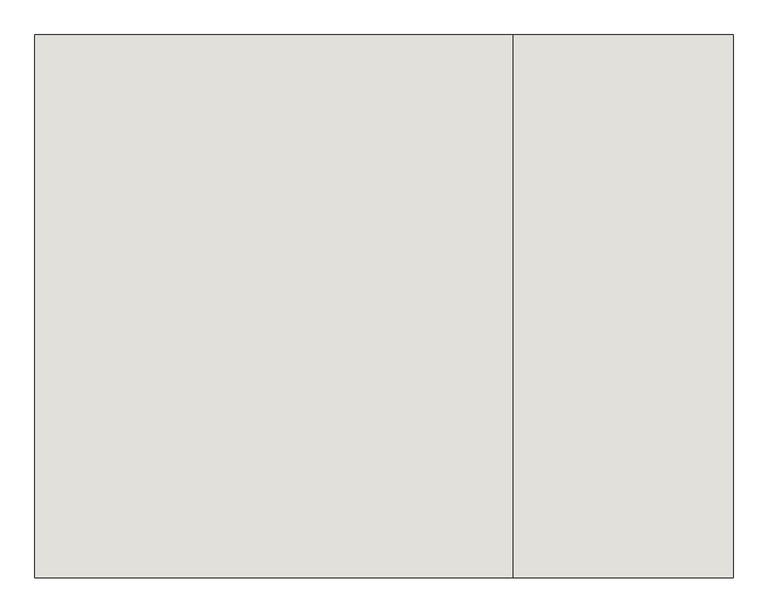
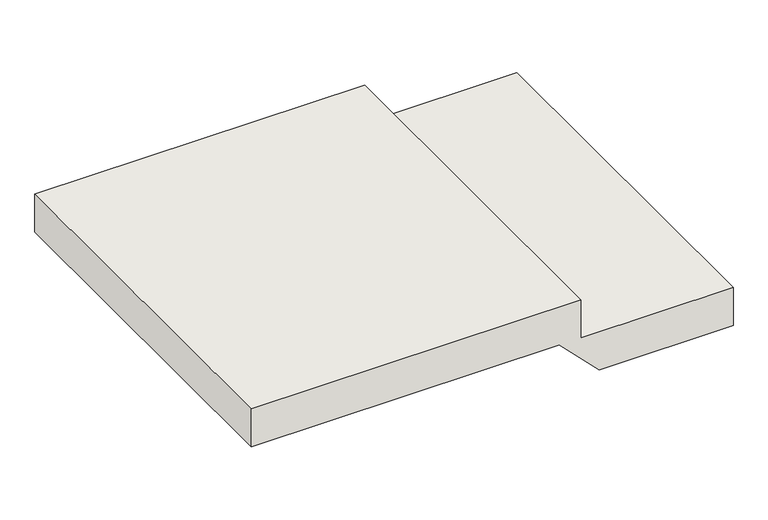
"""IFC4 building model written with IfcOpenShell, lengths in millimetres: wall geometry, 벽 5 : 벽 1."""

from ifc_helpers import new_model, si_unit, frame, origin, place, context, project, spatial, polyline, outline, extrude, source, transform, mapped, element, save


def wall_a06d278e(model_context):
    return source(origin(), model_context, "Body", "SweptSolid", [
        extrude(outline(polyline([(599.905241, 43602.1335861), (599.905241, 42370.0), (449.905241, 42370.0), (449.905241, 43520.0), (299.905241, 43670.0), (299.905241, 44170.4893475), (449.905241, 44170.4893475), (449.905241, 43602.1335861), (599.905241, 43602.1335861)])), frame((0.0, 21999.5208589, 0.0), z_axis=(0.0, 1.0, 0.0), x_axis=(0.0, 0.0, 1.0)), (0.0, 0.0, 1.0), 1400.0),
    ])


if __name__ == "__main__":
    model = new_model("IFC4")
    model_context = context("Model", 3, world=origin())
    ifc_project = project(units=[si_unit("LENGTHUNIT", "METRE", prefix="MILLI")], contexts=[model_context])
    site = spatial("IfcSite", under=ifc_project)
    building = spatial("IfcBuilding", under=site)
    placement = place(None, origin())
    wall_shape = wall_a06d278e(model_context)
    element("IfcWall", 1, ObjectType="벽 5 : 벽 1", at=placement, inside=building, context=model_context, shape_type="MappedRepresentation", body=[
        mapped(wall_shape, transform((0.0, 0.0, 0.0), x_axis=(1.0, 0.0, 0.0), y_axis=(0.0, 1.0, 0.0), z_axis=(0.0, 0.0, 1.0))),
    ])
    save(model, "model.ifc")

# Revit data of these elements
# Element 1 (IfcWall, "벽 5 : 벽 1")
#   Materials on its faces: "A03AC032-00007_Structural Concrete_Type1_25MPa-30Mpa"
# Materials
#   "A03AC032-00007_Structural Concrete_Type1_25MPa-30Mpa": class "Concrete", colour RGB 176 176 176, transparency 0, Keynote = "09910.A1", Description = "Reinf. Conc.", W00) Work Master Code = "A03AC032-00007", W01) Work Master_Lv1 = "Concrete Work", W02) Work Master_Lv2 = "Substructure Work", W03) Work Master_Spec.1 = "Structural Concrete", W04) Work Master_Spec.2 = "Cement Type-1", W05) Work Master_Spec.3 = "25MPa < F'c (Cylinder Strength) ≤ 30MPa", Cost = 0
